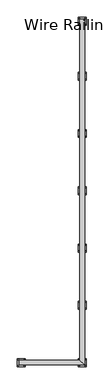
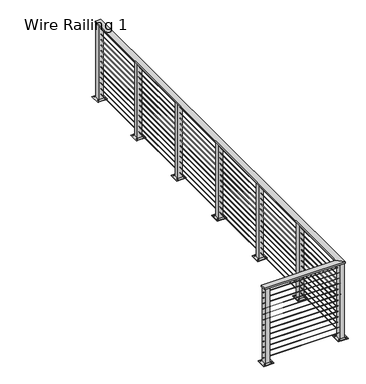
"""IFC4 building model written with IfcOpenShell, lengths in millimetres: railing geometry, Wire Railing 1."""

from ifc_helpers import new_model, si_unit, point, frame, frame_2d, origin, place, context, project, spatial, polyline, circle_curve, ellipse_curve, trimmed, segment, composite_curve, outline, extrude, faceted_brep, source, transform, mapped, element, save
from ifc_brep_helpers import plane_surface, cylinder_surface, advanced_brep


def wire_railing_1_7bc1b7ee(model_context):
    return source(origin(), model_context, "Body", "SolidModel", [
        faceted_brep([(33160.7531764, 36329.6332942, 267462.0), (33236.9531764, 36329.6332942, 267462.0), (33236.9531764, 36329.6332942, 267442.95), (33160.7531764, 36329.6332942, 267442.95), (33160.7531764, 30812.4406612, 267462.0), (33236.9531764, 30736.2406612, 267462.0), (33236.9531764, 30736.2406612, 267442.95), (33160.7531764, 30812.4406612, 267442.95), (32175.4465778, 30812.4406612, 267462.0), (32175.4465778, 30812.4406612, 267442.95), (32175.4465778, 30736.2406612, 267442.95), (32175.4465778, 30736.2406612, 267462.0)], [[[0, 1, 2, 3]], [[1, 0, 4, 5]], [[2, 1, 5, 6]], [[3, 2, 6, 7]], [[0, 3, 7, 4]], [[8, 9, 10, 11]], [[5, 4, 8, 11]], [[6, 5, 11, 10]], [[7, 6, 10, 9]], [[4, 7, 9, 8]]]),
        advanced_brep(
        [(33201.2344264, 36329.6332942, 267383.41875), (33196.4719264, 36329.6332942, 267383.41875), (33201.2344264, 30771.9594112, 267383.41875), (33196.4719264, 30776.7219112, 267383.41875), (32175.4465778, 30771.9594112, 267383.41875), (32175.4465778, 30776.7219112, 267383.41875)],
        [
            (0, 1, circle_curve(frame((33198.8531764, 36329.6332942, 267383.41875), z_axis=(0.0, 1.0, 0.0), x_axis=(-1.0, 0.0, 0.0)), 2.38125)),
            (1, 0, circle_curve(frame((33198.8531764, 36329.6332942, 267383.41875), z_axis=(0.0, 1.0, 0.0), x_axis=(-1.0, 0.0, 0.0)), 2.38125)),
            (0, 2),
            (2, 3, ellipse_curve(frame((33198.8531764, 30774.3406612, 267383.41875), z_axis=(0.7071067811865475, 0.7071067811865475, 0.0), x_axis=(-0.7071067811865474, 0.7071067811865476, 0.0)), 3.367596, 2.38125)),
            (3, 1),
            (3, 2, ellipse_curve(frame((33198.8531764, 30774.3406612, 267383.41875), z_axis=(0.7071067811865475, 0.7071067811865475, 0.0), x_axis=(-0.7071067811865474, 0.7071067811865476, 0.0)), 3.367596, 2.38125)),
            (4, 5, circle_curve(frame((32175.4465778, 30774.3406612, 267383.41875), z_axis=(-1.0, 0.0, 0.0), x_axis=(0.0, 1.0, 0.0)), 2.38125)),
            (5, 4, circle_curve(frame((32175.4465778, 30774.3406612, 267383.41875), z_axis=(-1.0, 0.0, 0.0), x_axis=(0.0, 1.0, 0.0)), 2.38125)),
            (2, 4),
            (5, 3),
        ],
        [
            plane_surface(frame((33198.8531764, 36329.6332942, 267385.8), z_axis=(0.0, 1.0, 0.0), x_axis=(0.0, 0.0, -1.0))),
            cylinder_surface(frame((33198.8531764, 36329.6332942, 267383.41875), z_axis=(0.0, 1.0, 0.0), x_axis=(-1.0, 0.0, 0.0)), 2.38125),
            plane_surface(frame((32175.4465778, 30774.3406612, 267385.8), z_axis=(-1.0, 0.0, 0.0), x_axis=(0.0, -1.0, 0.0))),
            cylinder_surface(frame((33198.8531764, 30774.3406612, 267383.41875), z_axis=(1.0, 0.0, 0.0), x_axis=(0.0, 1.0, 0.0)), 2.38125),
        ],
        [
            (0, [[1, 2]]),
            (1, [[-1, 3, 4, 5]]),
            (1, [[-2, -5, 6, -3]]),
            (2, [[7, 8]]),
            (3, [[-4, 9, -8, 10]]),
            (3, [[-6, -10, -7, -9]]),
        ],
    ),
        advanced_brep(
        [(33201.2344264, 36329.6332942, 267307.21875), (33196.4719264, 36329.6332942, 267307.21875), (33201.2344264, 30771.9594112, 267307.21875), (33196.4719264, 30776.7219112, 267307.21875), (32175.4465778, 30771.9594112, 267307.21875), (32175.4465778, 30776.7219112, 267307.21875)],
        [
            (0, 1, circle_curve(frame((33198.8531764, 36329.6332942, 267307.21875), z_axis=(0.0, 1.0, 0.0), x_axis=(-1.0, 0.0, 0.0)), 2.38125)),
            (1, 0, circle_curve(frame((33198.8531764, 36329.6332942, 267307.21875), z_axis=(0.0, 1.0, 0.0), x_axis=(-1.0, 0.0, 0.0)), 2.38125)),
            (0, 2),
            (2, 3, ellipse_curve(frame((33198.8531764, 30774.3406612, 267307.21875), z_axis=(0.7071067811865475, 0.7071067811865475, 0.0), x_axis=(-0.7071067811865474, 0.7071067811865476, 0.0)), 3.367596, 2.38125)),
            (3, 1),
            (3, 2, ellipse_curve(frame((33198.8531764, 30774.3406612, 267307.21875), z_axis=(0.7071067811865475, 0.7071067811865475, 0.0), x_axis=(-0.7071067811865474, 0.7071067811865476, 0.0)), 3.367596, 2.38125)),
            (4, 5, circle_curve(frame((32175.4465778, 30774.3406612, 267307.21875), z_axis=(-1.0, 0.0, 0.0), x_axis=(0.0, 1.0, 0.0)), 2.38125)),
            (5, 4, circle_curve(frame((32175.4465778, 30774.3406612, 267307.21875), z_axis=(-1.0, 0.0, 0.0), x_axis=(0.0, 1.0, 0.0)), 2.38125)),
            (2, 4),
            (5, 3),
        ],
        [
            plane_surface(frame((33198.8531764, 36329.6332942, 267309.6), z_axis=(0.0, 1.0, 0.0), x_axis=(0.0, 0.0, -1.0))),
            cylinder_surface(frame((33198.8531764, 36329.6332942, 267307.21875), z_axis=(0.0, 1.0, 0.0), x_axis=(-1.0, 0.0, 0.0)), 2.38125),
            plane_surface(frame((32175.4465778, 30774.3406612, 267309.6), z_axis=(-1.0, 0.0, 0.0), x_axis=(0.0, -1.0, 0.0))),
            cylinder_surface(frame((33198.8531764, 30774.3406612, 267307.21875), z_axis=(1.0, 0.0, 0.0), x_axis=(0.0, 1.0, 0.0)), 2.38125),
        ],
        [
            (0, [[1, 2]]),
            (1, [[-1, 3, 4, 5]]),
            (1, [[-2, -5, 6, -3]]),
            (2, [[7, 8]]),
            (3, [[-4, 9, -8, 10]]),
            (3, [[-6, -10, -7, -9]]),
        ],
    ),
        advanced_brep(
        [(33201.2344264, 36329.6332942, 267231.01875), (33196.4719264, 36329.6332942, 267231.01875), (33201.2344264, 30771.9594112, 267231.01875), (33196.4719264, 30776.7219112, 267231.01875), (32175.4465778, 30771.9594112, 267231.01875), (32175.4465778, 30776.7219112, 267231.01875)],
        [
            (0, 1, circle_curve(frame((33198.8531764, 36329.6332942, 267231.01875), z_axis=(0.0, 1.0, 0.0), x_axis=(-1.0, 0.0, 0.0)), 2.38125)),
            (1, 0, circle_curve(frame((33198.8531764, 36329.6332942, 267231.01875), z_axis=(0.0, 1.0, 0.0), x_axis=(-1.0, 0.0, 0.0)), 2.38125)),
            (0, 2),
            (2, 3, ellipse_curve(frame((33198.8531764, 30774.3406612, 267231.01875), z_axis=(0.7071067811865475, 0.7071067811865475, 0.0), x_axis=(-0.7071067811865474, 0.7071067811865476, 0.0)), 3.367596, 2.38125)),
            (3, 1),
            (3, 2, ellipse_curve(frame((33198.8531764, 30774.3406612, 267231.01875), z_axis=(0.7071067811865475, 0.7071067811865475, 0.0), x_axis=(-0.7071067811865474, 0.7071067811865476, 0.0)), 3.367596, 2.38125)),
            (4, 5, circle_curve(frame((32175.4465778, 30774.3406612, 267231.01875), z_axis=(-1.0, 0.0, 0.0), x_axis=(0.0, 1.0, 0.0)), 2.38125)),
            (5, 4, circle_curve(frame((32175.4465778, 30774.3406612, 267231.01875), z_axis=(-1.0, 0.0, 0.0), x_axis=(0.0, 1.0, 0.0)), 2.38125)),
            (2, 4),
            (5, 3),
        ],
        [
            plane_surface(frame((33198.8531764, 36329.6332942, 267233.4), z_axis=(0.0, 1.0, 0.0), x_axis=(0.0, 0.0, -1.0))),
            cylinder_surface(frame((33198.8531764, 36329.6332942, 267231.01875), z_axis=(0.0, 1.0, 0.0), x_axis=(-1.0, 0.0, 0.0)), 2.38125),
            plane_surface(frame((32175.4465778, 30774.3406612, 267233.4), z_axis=(-1.0, 0.0, 0.0), x_axis=(0.0, -1.0, 0.0))),
            cylinder_surface(frame((33198.8531764, 30774.3406612, 267231.01875), z_axis=(1.0, 0.0, 0.0), x_axis=(0.0, 1.0, 0.0)), 2.38125),
        ],
        [
            (0, [[1, 2]]),
            (1, [[-1, 3, 4, 5]]),
            (1, [[-2, -5, 6, -3]]),
            (2, [[7, 8]]),
            (3, [[-4, 9, -8, 10]]),
            (3, [[-6, -10, -7, -9]]),
        ],
    ),
        advanced_brep(
        [(33201.2344264, 36329.6332942, 267154.81875), (33196.4719264, 36329.6332942, 267154.81875), (33201.2344264, 30771.9594112, 267154.81875), (33196.4719264, 30776.7219112, 267154.81875), (32175.4465778, 30771.9594112, 267154.81875), (32175.4465778, 30776.7219112, 267154.81875)],
        [
            (0, 1, circle_curve(frame((33198.8531764, 36329.6332942, 267154.81875), z_axis=(0.0, 1.0, 0.0), x_axis=(-1.0, 0.0, 0.0)), 2.38125)),
            (1, 0, circle_curve(frame((33198.8531764, 36329.6332942, 267154.81875), z_axis=(0.0, 1.0, 0.0), x_axis=(-1.0, 0.0, 0.0)), 2.38125)),
            (0, 2),
            (2, 3, ellipse_curve(frame((33198.8531764, 30774.3406612, 267154.81875), z_axis=(0.7071067811865475, 0.7071067811865475, 0.0), x_axis=(-0.7071067811865474, 0.7071067811865476, 0.0)), 3.367596, 2.38125)),
            (3, 1),
            (3, 2, ellipse_curve(frame((33198.8531764, 30774.3406612, 267154.81875), z_axis=(0.7071067811865475, 0.7071067811865475, 0.0), x_axis=(-0.7071067811865474, 0.7071067811865476, 0.0)), 3.367596, 2.38125)),
            (4, 5, circle_curve(frame((32175.4465778, 30774.3406612, 267154.81875), z_axis=(-1.0, 0.0, 0.0), x_axis=(0.0, 1.0, 0.0)), 2.38125)),
            (5, 4, circle_curve(frame((32175.4465778, 30774.3406612, 267154.81875), z_axis=(-1.0, 0.0, 0.0), x_axis=(0.0, 1.0, 0.0)), 2.38125)),
            (2, 4),
            (5, 3),
        ],
        [
            plane_surface(frame((33198.8531764, 36329.6332942, 267157.2), z_axis=(0.0, 1.0, 0.0), x_axis=(0.0, 0.0, -1.0))),
            cylinder_surface(frame((33198.8531764, 36329.6332942, 267154.81875), z_axis=(0.0, 1.0, 0.0), x_axis=(-1.0, 0.0, 0.0)), 2.38125),
            plane_surface(frame((32175.4465778, 30774.3406612, 267157.2), z_axis=(-1.0, 0.0, 0.0), x_axis=(0.0, -1.0, 0.0))),
            cylinder_surface(frame((33198.8531764, 30774.3406612, 267154.81875), z_axis=(1.0, 0.0, 0.0), x_axis=(0.0, 1.0, 0.0)), 2.38125),
        ],
        [
            (0, [[1, 2]]),
            (1, [[-1, 3, 4, 5]]),
            (1, [[-2, -5, 6, -3]]),
            (2, [[7, 8]]),
            (3, [[-4, 9, -8, 10]]),
            (3, [[-6, -10, -7, -9]]),
        ],
    ),
        advanced_brep(
        [(33201.2344264, 36329.6332942, 267078.61875), (33196.4719264, 36329.6332942, 267078.61875), (33201.2344264, 30771.9594112, 267078.61875), (33196.4719264, 30776.7219112, 267078.61875), (32175.4465778, 30771.9594112, 267078.61875), (32175.4465778, 30776.7219112, 267078.61875)],
        [
            (0, 1, circle_curve(frame((33198.8531764, 36329.6332942, 267078.61875), z_axis=(0.0, 1.0, 0.0), x_axis=(-1.0, 0.0, 0.0)), 2.38125)),
            (1, 0, circle_curve(frame((33198.8531764, 36329.6332942, 267078.61875), z_axis=(0.0, 1.0, 0.0), x_axis=(-1.0, 0.0, 0.0)), 2.38125)),
            (0, 2),
            (2, 3, ellipse_curve(frame((33198.8531764, 30774.3406612, 267078.61875), z_axis=(0.7071067811865475, 0.7071067811865475, 0.0), x_axis=(-0.7071067811865474, 0.7071067811865476, 0.0)), 3.367596, 2.38125)),
            (3, 1),
            (3, 2, ellipse_curve(frame((33198.8531764, 30774.3406612, 267078.61875), z_axis=(0.7071067811865475, 0.7071067811865475, 0.0), x_axis=(-0.7071067811865474, 0.7071067811865476, 0.0)), 3.367596, 2.38125)),
            (4, 5, circle_curve(frame((32175.4465778, 30774.3406612, 267078.61875), z_axis=(-1.0, 0.0, 0.0), x_axis=(0.0, 1.0, 0.0)), 2.38125)),
            (5, 4, circle_curve(frame((32175.4465778, 30774.3406612, 267078.61875), z_axis=(-1.0, 0.0, 0.0), x_axis=(0.0, 1.0, 0.0)), 2.38125)),
            (2, 4),
            (5, 3),
        ],
        [
            plane_surface(frame((33198.8531764, 36329.6332942, 267081.0), z_axis=(0.0, 1.0, 0.0), x_axis=(0.0, 0.0, -1.0))),
            cylinder_surface(frame((33198.8531764, 36329.6332942, 267078.61875), z_axis=(0.0, 1.0, 0.0), x_axis=(-1.0, 0.0, 0.0)), 2.38125),
            plane_surface(frame((32175.4465778, 30774.3406612, 267081.0), z_axis=(-1.0, 0.0, 0.0), x_axis=(0.0, -1.0, 0.0))),
            cylinder_surface(frame((33198.8531764, 30774.3406612, 267078.61875), z_axis=(1.0, 0.0, 0.0), x_axis=(0.0, 1.0, 0.0)), 2.38125),
        ],
        [
            (0, [[1, 2]]),
            (1, [[-1, 3, 4, 5]]),
            (1, [[-2, -5, 6, -3]]),
            (2, [[7, 8]]),
            (3, [[-4, 9, -8, 10]]),
            (3, [[-6, -10, -7, -9]]),
        ],
    ),
        advanced_brep(
        [(33201.2344264, 36329.6332942, 267002.41875), (33196.4719264, 36329.6332942, 267002.41875), (33201.2344264, 30771.9594112, 267002.41875), (33196.4719264, 30776.7219112, 267002.41875), (32175.4465778, 30771.9594112, 267002.41875), (32175.4465778, 30776.7219112, 267002.41875)],
        [
            (0, 1, circle_curve(frame((33198.8531764, 36329.6332942, 267002.41875), z_axis=(0.0, 1.0, 0.0), x_axis=(-1.0, 0.0, 0.0)), 2.38125)),
            (1, 0, circle_curve(frame((33198.8531764, 36329.6332942, 267002.41875), z_axis=(0.0, 1.0, 0.0), x_axis=(-1.0, 0.0, 0.0)), 2.38125)),
            (0, 2),
            (2, 3, ellipse_curve(frame((33198.8531764, 30774.3406612, 267002.41875), z_axis=(0.7071067811865475, 0.7071067811865475, 0.0), x_axis=(-0.7071067811865474, 0.7071067811865476, 0.0)), 3.367596, 2.38125)),
            (3, 1),
            (3, 2, ellipse_curve(frame((33198.8531764, 30774.3406612, 267002.41875), z_axis=(0.7071067811865475, 0.7071067811865475, 0.0), x_axis=(-0.7071067811865474, 0.7071067811865476, 0.0)), 3.367596, 2.38125)),
            (4, 5, circle_curve(frame((32175.4465778, 30774.3406612, 267002.41875), z_axis=(-1.0, 0.0, 0.0), x_axis=(0.0, 1.0, 0.0)), 2.38125)),
            (5, 4, circle_curve(frame((32175.4465778, 30774.3406612, 267002.41875), z_axis=(-1.0, 0.0, 0.0), x_axis=(0.0, 1.0, 0.0)), 2.38125)),
            (2, 4),
            (5, 3),
        ],
        [
            plane_surface(frame((33198.8531764, 36329.6332942, 267004.8), z_axis=(0.0, 1.0, 0.0), x_axis=(0.0, 0.0, -1.0))),
            cylinder_surface(frame((33198.8531764, 36329.6332942, 267002.41875), z_axis=(0.0, 1.0, 0.0), x_axis=(-1.0, 0.0, 0.0)), 2.38125),
            plane_surface(frame((32175.4465778, 30774.3406612, 267004.8), z_axis=(-1.0, 0.0, 0.0), x_axis=(0.0, -1.0, 0.0))),
            cylinder_surface(frame((33198.8531764, 30774.3406612, 267002.41875), z_axis=(1.0, 0.0, 0.0), x_axis=(0.0, 1.0, 0.0)), 2.38125),
        ],
        [
            (0, [[1, 2]]),
            (1, [[-1, 3, 4, 5]]),
            (1, [[-2, -5, 6, -3]]),
            (2, [[7, 8]]),
            (3, [[-4, 9, -8, 10]]),
            (3, [[-6, -10, -7, -9]]),
        ],
    ),
        advanced_brep(
        [(33201.2344264, 36329.6332942, 266926.21875), (33196.4719264, 36329.6332942, 266926.21875), (33201.2344264, 30771.9594112, 266926.21875), (33196.4719264, 30776.7219112, 266926.21875), (32175.4465778, 30771.9594112, 266926.21875), (32175.4465778, 30776.7219112, 266926.21875)],
        [
            (0, 1, circle_curve(frame((33198.8531764, 36329.6332942, 266926.21875), z_axis=(0.0, 1.0, 0.0), x_axis=(-1.0, 0.0, 0.0)), 2.38125)),
            (1, 0, circle_curve(frame((33198.8531764, 36329.6332942, 266926.21875), z_axis=(0.0, 1.0, 0.0), x_axis=(-1.0, 0.0, 0.0)), 2.38125)),
            (0, 2),
            (2, 3, ellipse_curve(frame((33198.8531764, 30774.3406612, 266926.21875), z_axis=(0.7071067811865475, 0.7071067811865475, 0.0), x_axis=(-0.7071067811865474, 0.7071067811865476, 0.0)), 3.367596, 2.38125)),
            (3, 1),
            (3, 2, ellipse_curve(frame((33198.8531764, 30774.3406612, 266926.21875), z_axis=(0.7071067811865475, 0.7071067811865475, 0.0), x_axis=(-0.7071067811865474, 0.7071067811865476, 0.0)), 3.367596, 2.38125)),
            (4, 5, circle_curve(frame((32175.4465778, 30774.3406612, 266926.21875), z_axis=(-1.0, 0.0, 0.0), x_axis=(0.0, 1.0, 0.0)), 2.38125)),
            (5, 4, circle_curve(frame((32175.4465778, 30774.3406612, 266926.21875), z_axis=(-1.0, 0.0, 0.0), x_axis=(0.0, 1.0, 0.0)), 2.38125)),
            (2, 4),
            (5, 3),
        ],
        [
            plane_surface(frame((33198.8531764, 36329.6332942, 266928.6), z_axis=(0.0, 1.0, 0.0), x_axis=(0.0, 0.0, -1.0))),
            cylinder_surface(frame((33198.8531764, 36329.6332942, 266926.21875), z_axis=(0.0, 1.0, 0.0), x_axis=(-1.0, 0.0, 0.0)), 2.38125),
            plane_surface(frame((32175.4465778, 30774.3406612, 266928.6), z_axis=(-1.0, 0.0, 0.0), x_axis=(0.0, -1.0, 0.0))),
            cylinder_surface(frame((33198.8531764, 30774.3406612, 266926.21875), z_axis=(1.0, 0.0, 0.0), x_axis=(0.0, 1.0, 0.0)), 2.38125),
        ],
        [
            (0, [[1, 2]]),
            (1, [[-1, 3, 4, 5]]),
            (1, [[-2, -5, 6, -3]]),
            (2, [[7, 8]]),
            (3, [[-4, 9, -8, 10]]),
            (3, [[-6, -10, -7, -9]]),
        ],
    ),
        advanced_brep(
        [(33201.2344264, 36329.6332942, 266850.01875), (33196.4719264, 36329.6332942, 266850.01875), (33201.2344264, 30771.9594112, 266850.01875), (33196.4719264, 30776.7219112, 266850.01875), (32175.4465778, 30771.9594112, 266850.01875), (32175.4465778, 30776.7219112, 266850.01875)],
        [
            (0, 1, circle_curve(frame((33198.8531764, 36329.6332942, 266850.01875), z_axis=(0.0, 1.0, 0.0), x_axis=(-1.0, 0.0, 0.0)), 2.38125)),
            (1, 0, circle_curve(frame((33198.8531764, 36329.6332942, 266850.01875), z_axis=(0.0, 1.0, 0.0), x_axis=(-1.0, 0.0, 0.0)), 2.38125)),
            (0, 2),
            (2, 3, ellipse_curve(frame((33198.8531764, 30774.3406612, 266850.01875), z_axis=(0.7071067811865475, 0.7071067811865475, 0.0), x_axis=(-0.7071067811865474, 0.7071067811865476, 0.0)), 3.367596, 2.38125)),
            (3, 1),
            (3, 2, ellipse_curve(frame((33198.8531764, 30774.3406612, 266850.01875), z_axis=(0.7071067811865475, 0.7071067811865475, 0.0), x_axis=(-0.7071067811865474, 0.7071067811865476, 0.0)), 3.367596, 2.38125)),
            (4, 5, circle_curve(frame((32175.4465778, 30774.3406612, 266850.01875), z_axis=(-1.0, 0.0, 0.0), x_axis=(0.0, 1.0, 0.0)), 2.38125)),
            (5, 4, circle_curve(frame((32175.4465778, 30774.3406612, 266850.01875), z_axis=(-1.0, 0.0, 0.0), x_axis=(0.0, 1.0, 0.0)), 2.38125)),
            (2, 4),
            (5, 3),
        ],
        [
            plane_surface(frame((33198.8531764, 36329.6332942, 266852.4), z_axis=(0.0, 1.0, 0.0), x_axis=(0.0, 0.0, -1.0))),
            cylinder_surface(frame((33198.8531764, 36329.6332942, 266850.01875), z_axis=(0.0, 1.0, 0.0), x_axis=(-1.0, 0.0, 0.0)), 2.38125),
            plane_surface(frame((32175.4465778, 30774.3406612, 266852.4), z_axis=(-1.0, 0.0, 0.0), x_axis=(0.0, -1.0, 0.0))),
            cylinder_surface(frame((33198.8531764, 30774.3406612, 266850.01875), z_axis=(1.0, 0.0, 0.0), x_axis=(0.0, 1.0, 0.0)), 2.38125),
        ],
        [
            (0, [[1, 2]]),
            (1, [[-1, 3, 4, 5]]),
            (1, [[-2, -5, 6, -3]]),
            (2, [[7, 8]]),
            (3, [[-4, 9, -8, 10]]),
            (3, [[-6, -10, -7, -9]]),
        ],
    ),
        advanced_brep(
        [(33201.2344264, 36329.6332942, 266773.81875), (33196.4719264, 36329.6332942, 266773.81875), (33201.2344264, 30771.9594112, 266773.81875), (33196.4719264, 30776.7219112, 266773.81875), (32175.4465778, 30771.9594112, 266773.81875), (32175.4465778, 30776.7219112, 266773.81875)],
        [
            (0, 1, circle_curve(frame((33198.8531764, 36329.6332942, 266773.81875), z_axis=(0.0, 1.0, 0.0), x_axis=(-1.0, 0.0, 0.0)), 2.38125)),
            (1, 0, circle_curve(frame((33198.8531764, 36329.6332942, 266773.81875), z_axis=(0.0, 1.0, 0.0), x_axis=(-1.0, 0.0, 0.0)), 2.38125)),
            (0, 2),
            (2, 3, ellipse_curve(frame((33198.8531764, 30774.3406612, 266773.81875), z_axis=(0.7071067811865475, 0.7071067811865475, 0.0), x_axis=(-0.7071067811865474, 0.7071067811865476, 0.0)), 3.367596, 2.38125)),
            (3, 1),
            (3, 2, ellipse_curve(frame((33198.8531764, 30774.3406612, 266773.81875), z_axis=(0.7071067811865475, 0.7071067811865475, 0.0), x_axis=(-0.7071067811865474, 0.7071067811865476, 0.0)), 3.367596, 2.38125)),
            (4, 5, circle_curve(frame((32175.4465778, 30774.3406612, 266773.81875), z_axis=(-1.0, 0.0, 0.0), x_axis=(0.0, 1.0, 0.0)), 2.38125)),
            (5, 4, circle_curve(frame((32175.4465778, 30774.3406612, 266773.81875), z_axis=(-1.0, 0.0, 0.0), x_axis=(0.0, 1.0, 0.0)), 2.38125)),
            (2, 4),
            (5, 3),
        ],
        [
            plane_surface(frame((33198.8531764, 36329.6332942, 266776.2), z_axis=(0.0, 1.0, 0.0), x_axis=(0.0, 0.0, -1.0))),
            cylinder_surface(frame((33198.8531764, 36329.6332942, 266773.81875), z_axis=(0.0, 1.0, 0.0), x_axis=(-1.0, 0.0, 0.0)), 2.38125),
            plane_surface(frame((32175.4465778, 30774.3406612, 266776.2), z_axis=(-1.0, 0.0, 0.0), x_axis=(0.0, -1.0, 0.0))),
            cylinder_surface(frame((33198.8531764, 30774.3406612, 266773.81875), z_axis=(1.0, 0.0, 0.0), x_axis=(0.0, 1.0, 0.0)), 2.38125),
        ],
        [
            (0, [[1, 2]]),
            (1, [[-1, 3, 4, 5]]),
            (1, [[-2, -5, 6, -3]]),
            (2, [[7, 8]]),
            (3, [[-4, 9, -8, 10]]),
            (3, [[-6, -10, -7, -9]]),
        ],
    ),
        advanced_brep(
        [(33201.2344264, 36329.6332942, 266697.61875), (33196.4719264, 36329.6332942, 266697.61875), (33201.2344264, 30771.9594112, 266697.61875), (33196.4719264, 30776.7219112, 266697.61875), (32175.4465778, 30771.9594112, 266697.61875), (32175.4465778, 30776.7219112, 266697.61875)],
        [
            (0, 1, circle_curve(frame((33198.8531764, 36329.6332942, 266697.61875), z_axis=(0.0, 1.0, 0.0), x_axis=(-1.0, 0.0, 0.0)), 2.38125)),
            (1, 0, circle_curve(frame((33198.8531764, 36329.6332942, 266697.61875), z_axis=(0.0, 1.0, 0.0), x_axis=(-1.0, 0.0, 0.0)), 2.38125)),
            (0, 2),
            (2, 3, ellipse_curve(frame((33198.8531764, 30774.3406612, 266697.61875), z_axis=(0.7071067811865475, 0.7071067811865475, 0.0), x_axis=(-0.7071067811865474, 0.7071067811865476, 0.0)), 3.367596, 2.38125)),
            (3, 1),
            (3, 2, ellipse_curve(frame((33198.8531764, 30774.3406612, 266697.61875), z_axis=(0.7071067811865475, 0.7071067811865475, 0.0), x_axis=(-0.7071067811865474, 0.7071067811865476, 0.0)), 3.367596, 2.38125)),
            (4, 5, circle_curve(frame((32175.4465778, 30774.3406612, 266697.61875), z_axis=(-1.0, 0.0, 0.0), x_axis=(0.0, 1.0, 0.0)), 2.38125)),
            (5, 4, circle_curve(frame((32175.4465778, 30774.3406612, 266697.61875), z_axis=(-1.0, 0.0, 0.0), x_axis=(0.0, 1.0, 0.0)), 2.38125)),
            (2, 4),
            (5, 3),
        ],
        [
            plane_surface(frame((33198.8531764, 36329.6332942, 266700.0), z_axis=(0.0, 1.0, 0.0), x_axis=(0.0, 0.0, -1.0))),
            cylinder_surface(frame((33198.8531764, 36329.6332942, 266697.61875), z_axis=(0.0, 1.0, 0.0), x_axis=(-1.0, 0.0, 0.0)), 2.38125),
            plane_surface(frame((32175.4465778, 30774.3406612, 266700.0), z_axis=(-1.0, 0.0, 0.0), x_axis=(0.0, -1.0, 0.0))),
            cylinder_surface(frame((33198.8531764, 30774.3406612, 266697.61875), z_axis=(1.0, 0.0, 0.0), x_axis=(0.0, 1.0, 0.0)), 2.38125),
        ],
        [
            (0, [[1, 2]]),
            (1, [[-1, 3, 4, 5]]),
            (1, [[-2, -5, 6, -3]]),
            (2, [[7, 8]]),
            (3, [[-4, 9, -8, 10]]),
            (3, [[-6, -10, -7, -9]]),
        ],
    ),
        advanced_brep(
        [(33201.2344264, 36329.6332942, 266621.41875), (33196.4719264, 36329.6332942, 266621.41875), (33201.2344264, 30771.9594112, 266621.41875), (33196.4719264, 30776.7219112, 266621.41875), (32175.4465778, 30771.9594112, 266621.41875), (32175.4465778, 30776.7219112, 266621.41875)],
        [
            (0, 1, circle_curve(frame((33198.8531764, 36329.6332942, 266621.41875), z_axis=(0.0, 1.0, 0.0), x_axis=(-1.0, 0.0, 0.0)), 2.38125)),
            (1, 0, circle_curve(frame((33198.8531764, 36329.6332942, 266621.41875), z_axis=(0.0, 1.0, 0.0), x_axis=(-1.0, 0.0, 0.0)), 2.38125)),
            (0, 2),
            (2, 3, ellipse_curve(frame((33198.8531764, 30774.3406612, 266621.41875), z_axis=(0.7071067811865475, 0.7071067811865475, 0.0), x_axis=(-0.7071067811865474, 0.7071067811865476, 0.0)), 3.367596, 2.38125)),
            (3, 1),
            (3, 2, ellipse_curve(frame((33198.8531764, 30774.3406612, 266621.41875), z_axis=(0.7071067811865475, 0.7071067811865475, 0.0), x_axis=(-0.7071067811865474, 0.7071067811865476, 0.0)), 3.367596, 2.38125)),
            (4, 5, circle_curve(frame((32175.4465778, 30774.3406612, 266621.41875), z_axis=(-1.0, 0.0, 0.0), x_axis=(0.0, 1.0, 0.0)), 2.38125)),
            (5, 4, circle_curve(frame((32175.4465778, 30774.3406612, 266621.41875), z_axis=(-1.0, 0.0, 0.0), x_axis=(0.0, 1.0, 0.0)), 2.38125)),
            (2, 4),
            (5, 3),
        ],
        [
            plane_surface(frame((33198.8531764, 36329.6332942, 266623.8), z_axis=(0.0, 1.0, 0.0), x_axis=(0.0, 0.0, -1.0))),
            cylinder_surface(frame((33198.8531764, 36329.6332942, 266621.41875), z_axis=(0.0, 1.0, 0.0), x_axis=(-1.0, 0.0, 0.0)), 2.38125),
            plane_surface(frame((32175.4465778, 30774.3406612, 266623.8), z_axis=(-1.0, 0.0, 0.0), x_axis=(0.0, -1.0, 0.0))),
            cylinder_surface(frame((33198.8531764, 30774.3406612, 266621.41875), z_axis=(1.0, 0.0, 0.0), x_axis=(0.0, 1.0, 0.0)), 2.38125),
        ],
        [
            (0, [[1, 2]]),
            (1, [[-1, 3, 4, 5]]),
            (1, [[-2, -5, 6, -3]]),
            (2, [[7, 8]]),
            (3, [[-4, 9, -8, 10]]),
            (3, [[-6, -10, -7, -9]]),
        ],
    ),
        advanced_brep(
        [(33201.2344264, 36329.6332942, 266545.21875), (33196.4719264, 36329.6332942, 266545.21875), (33201.2344264, 30771.9594112, 266545.21875), (33196.4719264, 30776.7219112, 266545.21875), (32175.4465778, 30771.9594112, 266545.21875), (32175.4465778, 30776.7219112, 266545.21875)],
        [
            (0, 1, circle_curve(frame((33198.8531764, 36329.6332942, 266545.21875), z_axis=(0.0, 1.0, 0.0), x_axis=(-1.0, 0.0, 0.0)), 2.38125)),
            (1, 0, circle_curve(frame((33198.8531764, 36329.6332942, 266545.21875), z_axis=(0.0, 1.0, 0.0), x_axis=(-1.0, 0.0, 0.0)), 2.38125)),
            (0, 2),
            (2, 3, ellipse_curve(frame((33198.8531764, 30774.3406612, 266545.21875), z_axis=(0.7071067811865475, 0.7071067811865475, 0.0), x_axis=(-0.7071067811865474, 0.7071067811865476, 0.0)), 3.367596, 2.38125)),
            (3, 1),
            (3, 2, ellipse_curve(frame((33198.8531764, 30774.3406612, 266545.21875), z_axis=(0.7071067811865475, 0.7071067811865475, 0.0), x_axis=(-0.7071067811865474, 0.7071067811865476, 0.0)), 3.367596, 2.38125)),
            (4, 5, circle_curve(frame((32175.4465778, 30774.3406612, 266545.21875), z_axis=(-1.0, 0.0, 0.0), x_axis=(0.0, 1.0, 0.0)), 2.38125)),
            (5, 4, circle_curve(frame((32175.4465778, 30774.3406612, 266545.21875), z_axis=(-1.0, 0.0, 0.0), x_axis=(0.0, 1.0, 0.0)), 2.38125)),
            (2, 4),
            (5, 3),
        ],
        [
            plane_surface(frame((33198.8531764, 36329.6332942, 266547.6), z_axis=(0.0, 1.0, 0.0), x_axis=(0.0, 0.0, -1.0))),
            cylinder_surface(frame((33198.8531764, 36329.6332942, 266545.21875), z_axis=(0.0, 1.0, 0.0), x_axis=(-1.0, 0.0, 0.0)), 2.38125),
            plane_surface(frame((32175.4465778, 30774.3406612, 266547.6), z_axis=(-1.0, 0.0, 0.0), x_axis=(0.0, -1.0, 0.0))),
            cylinder_surface(frame((33198.8531764, 30774.3406612, 266545.21875), z_axis=(1.0, 0.0, 0.0), x_axis=(0.0, 1.0, 0.0)), 2.38125),
        ],
        [
            (0, [[1, 2]]),
            (1, [[-1, 3, 4, 5]]),
            (1, [[-2, -5, 6, -3]]),
            (2, [[7, 8]]),
            (3, [[-4, 9, -8, 10]]),
            (3, [[-6, -10, -7, -9]]),
        ],
    ),
        advanced_brep(
        [(33201.2344264, 36329.6332942, 266469.01875), (33196.4719264, 36329.6332942, 266469.01875), (33201.2344264, 30771.9594112, 266469.01875), (33196.4719264, 30776.7219112, 266469.01875), (32175.4465778, 30771.9594112, 266469.01875), (32175.4465778, 30776.7219112, 266469.01875)],
        [
            (0, 1, circle_curve(frame((33198.8531764, 36329.6332942, 266469.01875), z_axis=(0.0, 1.0, 0.0), x_axis=(-1.0, 0.0, 0.0)), 2.38125)),
            (1, 0, circle_curve(frame((33198.8531764, 36329.6332942, 266469.01875), z_axis=(0.0, 1.0, 0.0), x_axis=(-1.0, 0.0, 0.0)), 2.38125)),
            (0, 2),
            (2, 3, ellipse_curve(frame((33198.8531764, 30774.3406612, 266469.01875), z_axis=(0.7071067811865475, 0.7071067811865475, 0.0), x_axis=(-0.7071067811865474, 0.7071067811865476, 0.0)), 3.367596, 2.38125)),
            (3, 1),
            (3, 2, ellipse_curve(frame((33198.8531764, 30774.3406612, 266469.01875), z_axis=(0.7071067811865475, 0.7071067811865475, 0.0), x_axis=(-0.7071067811865474, 0.7071067811865476, 0.0)), 3.367596, 2.38125)),
            (4, 5, circle_curve(frame((32175.4465778, 30774.3406612, 266469.01875), z_axis=(-1.0, 0.0, 0.0), x_axis=(0.0, 1.0, 0.0)), 2.38125)),
            (5, 4, circle_curve(frame((32175.4465778, 30774.3406612, 266469.01875), z_axis=(-1.0, 0.0, 0.0), x_axis=(0.0, 1.0, 0.0)), 2.38125)),
            (2, 4),
            (5, 3),
        ],
        [
            plane_surface(frame((33198.8531764, 36329.6332942, 266471.4), z_axis=(0.0, 1.0, 0.0), x_axis=(0.0, 0.0, -1.0))),
            cylinder_surface(frame((33198.8531764, 36329.6332942, 266469.01875), z_axis=(0.0, 1.0, 0.0), x_axis=(-1.0, 0.0, 0.0)), 2.38125),
            plane_surface(frame((32175.4465778, 30774.3406612, 266471.4), z_axis=(-1.0, 0.0, 0.0), x_axis=(0.0, -1.0, 0.0))),
            cylinder_surface(frame((33198.8531764, 30774.3406612, 266469.01875), z_axis=(1.0, 0.0, 0.0), x_axis=(0.0, 1.0, 0.0)), 2.38125),
        ],
        [
            (0, [[1, 2]]),
            (1, [[-1, 3, 4, 5]]),
            (1, [[-2, -5, 6, -3]]),
            (2, [[7, 8]]),
            (3, [[-4, 9, -8, 10]]),
            (3, [[-6, -10, -7, -9]]),
        ],
    ),
        extrude(outline(composite_curve([segment(trimmed(circle_curve(frame_2d((33154.4031764, 31744.6727667)), 6.35), [point((33148.0531764, 31744.6727667))], [point((33160.7531764, 31744.6727667))], False, "CARTESIAN"), True, "CONTINUOUS"), segment(trimmed(circle_curve(frame_2d((33154.4031764, 31744.6727667)), 6.35), [point((33160.7531764, 31744.6727667))], [point((33148.0531764, 31744.6727667))], False, "CARTESIAN"), True, "CONTINUOUS")], self_intersect=False)), frame((0.0, 0.0, 266395.2), z_axis=(0.0, 0.0, 1.0), x_axis=(1.0, 0.0, 0.0)), (0.0, 0.0, 1.0), 12.7),
        extrude(outline(composite_curve([segment(trimmed(circle_curve(frame_2d((33243.3031764, 31744.6727667)), 6.35), [point((33236.9531764, 31744.6727667))], [point((33249.6531764, 31744.6727667))], False, "CARTESIAN"), True, "CONTINUOUS"), segment(trimmed(circle_curve(frame_2d((33243.3031764, 31744.6727667)), 6.35), [point((33249.6531764, 31744.6727667))], [point((33236.9531764, 31744.6727667))], False, "CARTESIAN"), True, "CONTINUOUS")], self_intersect=False)), frame((0.0, 0.0, 266395.2), z_axis=(0.0, 0.0, 1.0), x_axis=(1.0, 0.0, 0.0)), (0.0, 0.0, 1.0), 12.7),
        extrude(outline(composite_curve([segment(trimmed(circle_curve(frame_2d((33154.4031764, 31655.7727667)), 6.35), [point((33148.0531764, 31655.7727667))], [point((33160.7531764, 31655.7727667))], False, "CARTESIAN"), True, "CONTINUOUS"), segment(trimmed(circle_curve(frame_2d((33154.4031764, 31655.7727667)), 6.35), [point((33160.7531764, 31655.7727667))], [point((33148.0531764, 31655.7727667))], False, "CARTESIAN"), True, "CONTINUOUS")], self_intersect=False)), frame((0.0, 0.0, 266395.2), z_axis=(0.0, 0.0, 1.0), x_axis=(1.0, 0.0, 0.0)), (0.0, 0.0, 1.0), 12.7),
        extrude(outline(composite_curve([segment(trimmed(circle_curve(frame_2d((33243.3031764, 31655.7727667)), 6.35), [point((33236.9531764, 31655.7727667))], [point((33249.6531764, 31655.7727667))], False, "CARTESIAN"), True, "CONTINUOUS"), segment(trimmed(circle_curve(frame_2d((33243.3031764, 31655.7727667)), 6.35), [point((33249.6531764, 31655.7727667))], [point((33236.9531764, 31655.7727667))], False, "CARTESIAN"), True, "CONTINUOUS")], self_intersect=False)), frame((0.0, 0.0, 266395.2), z_axis=(0.0, 0.0, 1.0), x_axis=(1.0, 0.0, 0.0)), (0.0, 0.0, 1.0), 12.7),
        extrude(outline(polyline([(33262.3531764, 31763.7227667), (33262.3531764, 31636.7227667), (33135.3531764, 31636.7227667), (33135.3531764, 31763.7227667), (33262.3531764, 31763.7227667)])), frame((0.0, 0.0, 266395.2), z_axis=(0.0, 0.0, 1.0), x_axis=(1.0, 0.0, 0.0)), (0.0, 0.0, 1.0), 6.35),
        extrude(outline(polyline([(33229.0156764, 31730.3852667), (33229.0156764, 31670.0602667), (33168.6906764, 31670.0602667), (33168.6906764, 31730.3852667), (33229.0156764, 31730.3852667)]), holes=[polyline([(33222.6656764, 31724.0352667), (33175.0406764, 31724.0352667), (33175.0406764, 31676.4102667), (33222.6656764, 31676.4102667), (33222.6656764, 31724.0352667)])]), frame((0.0, 0.0, 266395.2), z_axis=(0.0, 0.0, 1.0), x_axis=(1.0, 0.0, 0.0)), (0.0, 0.0, 1.0), 1047.75),
        extrude(outline(composite_curve([segment(trimmed(circle_curve(frame_2d((33154.4031764, 32670.5548722)), 6.35), [point((33148.0531764, 32670.5548722))], [point((33160.7531764, 32670.5548722))], False, "CARTESIAN"), True, "CONTINUOUS"), segment(trimmed(circle_curve(frame_2d((33154.4031764, 32670.5548722)), 6.35), [point((33160.7531764, 32670.5548722))], [point((33148.0531764, 32670.5548722))], False, "CARTESIAN"), True, "CONTINUOUS")], self_intersect=False)), frame((0.0, 0.0, 266395.2), z_axis=(0.0, 0.0, 1.0), x_axis=(1.0, 0.0, 0.0)), (0.0, 0.0, 1.0), 12.7),
        extrude(outline(composite_curve([segment(trimmed(circle_curve(frame_2d((33243.3031764, 32670.5548722)), 6.35), [point((33236.9531764, 32670.5548722))], [point((33249.6531764, 32670.5548722))], False, "CARTESIAN"), True, "CONTINUOUS"), segment(trimmed(circle_curve(frame_2d((33243.3031764, 32670.5548722)), 6.35), [point((33249.6531764, 32670.5548722))], [point((33236.9531764, 32670.5548722))], False, "CARTESIAN"), True, "CONTINUOUS")], self_intersect=False)), frame((0.0, 0.0, 266395.2), z_axis=(0.0, 0.0, 1.0), x_axis=(1.0, 0.0, 0.0)), (0.0, 0.0, 1.0), 12.7),
        extrude(outline(composite_curve([segment(trimmed(circle_curve(frame_2d((33154.4031764, 32581.6548722)), 6.35), [point((33148.0531764, 32581.6548722))], [point((33160.7531764, 32581.6548722))], False, "CARTESIAN"), True, "CONTINUOUS"), segment(trimmed(circle_curve(frame_2d((33154.4031764, 32581.6548722)), 6.35), [point((33160.7531764, 32581.6548722))], [point((33148.0531764, 32581.6548722))], False, "CARTESIAN"), True, "CONTINUOUS")], self_intersect=False)), frame((0.0, 0.0, 266395.2), z_axis=(0.0, 0.0, 1.0), x_axis=(1.0, 0.0, 0.0)), (0.0, 0.0, 1.0), 12.7),
        extrude(outline(composite_curve([segment(trimmed(circle_curve(frame_2d((33243.3031764, 32581.6548722)), 6.35), [point((33236.9531764, 32581.6548722))], [point((33249.6531764, 32581.6548722))], False, "CARTESIAN"), True, "CONTINUOUS"), segment(trimmed(circle_curve(frame_2d((33243.3031764, 32581.6548722)), 6.35), [point((33249.6531764, 32581.6548722))], [point((33236.9531764, 32581.6548722))], False, "CARTESIAN"), True, "CONTINUOUS")], self_intersect=False)), frame((0.0, 0.0, 266395.2), z_axis=(0.0, 0.0, 1.0), x_axis=(1.0, 0.0, 0.0)), (0.0, 0.0, 1.0), 12.7),
        extrude(outline(polyline([(33262.3531764, 32689.6048722), (33262.3531764, 32562.6048722), (33135.3531764, 32562.6048722), (33135.3531764, 32689.6048722), (33262.3531764, 32689.6048722)])), frame((0.0, 0.0, 266395.2), z_axis=(0.0, 0.0, 1.0), x_axis=(1.0, 0.0, 0.0)), (0.0, 0.0, 1.0), 6.35),
        extrude(outline(polyline([(33229.0156764, 32656.2673722), (33229.0156764, 32595.9423722), (33168.6906764, 32595.9423722), (33168.6906764, 32656.2673722), (33229.0156764, 32656.2673722)]), holes=[polyline([(33222.6656764, 32649.9173722), (33175.0406764, 32649.9173722), (33175.0406764, 32602.2923722), (33222.6656764, 32602.2923722), (33222.6656764, 32649.9173722)])]), frame((0.0, 0.0, 266395.2), z_axis=(0.0, 0.0, 1.0), x_axis=(1.0, 0.0, 0.0)), (0.0, 0.0, 1.0), 1047.75),
        extrude(outline(composite_curve([segment(trimmed(circle_curve(frame_2d((33154.4031764, 33596.4369777)), 6.35), [point((33148.0531764, 33596.4369777))], [point((33160.7531764, 33596.4369777))], False, "CARTESIAN"), True, "CONTINUOUS"), segment(trimmed(circle_curve(frame_2d((33154.4031764, 33596.4369777)), 6.35), [point((33160.7531764, 33596.4369777))], [point((33148.0531764, 33596.4369777))], False, "CARTESIAN"), True, "CONTINUOUS")], self_intersect=False)), frame((0.0, 0.0, 266395.2), z_axis=(0.0, 0.0, 1.0), x_axis=(1.0, 0.0, 0.0)), (0.0, 0.0, 1.0), 12.7),
        extrude(outline(composite_curve([segment(trimmed(circle_curve(frame_2d((33243.3031764, 33596.4369777)), 6.35), [point((33236.9531764, 33596.4369777))], [point((33249.6531764, 33596.4369777))], False, "CARTESIAN"), True, "CONTINUOUS"), segment(trimmed(circle_curve(frame_2d((33243.3031764, 33596.4369777)), 6.35), [point((33249.6531764, 33596.4369777))], [point((33236.9531764, 33596.4369777))], False, "CARTESIAN"), True, "CONTINUOUS")], self_intersect=False)), frame((0.0, 0.0, 266395.2), z_axis=(0.0, 0.0, 1.0), x_axis=(1.0, 0.0, 0.0)), (0.0, 0.0, 1.0), 12.7),
        extrude(outline(composite_curve([segment(trimmed(circle_curve(frame_2d((33154.4031764, 33507.5369777)), 6.35), [point((33148.0531764, 33507.5369777))], [point((33160.7531764, 33507.5369777))], False, "CARTESIAN"), True, "CONTINUOUS"), segment(trimmed(circle_curve(frame_2d((33154.4031764, 33507.5369777)), 6.35), [point((33160.7531764, 33507.5369777))], [point((33148.0531764, 33507.5369777))], False, "CARTESIAN"), True, "CONTINUOUS")], self_intersect=False)), frame((0.0, 0.0, 266395.2), z_axis=(0.0, 0.0, 1.0), x_axis=(1.0, 0.0, 0.0)), (0.0, 0.0, 1.0), 12.7),
        extrude(outline(composite_curve([segment(trimmed(circle_curve(frame_2d((33243.3031764, 33507.5369777)), 6.35), [point((33236.9531764, 33507.5369777))], [point((33249.6531764, 33507.5369777))], False, "CARTESIAN"), True, "CONTINUOUS"), segment(trimmed(circle_curve(frame_2d((33243.3031764, 33507.5369777)), 6.35), [point((33249.6531764, 33507.5369777))], [point((33236.9531764, 33507.5369777))], False, "CARTESIAN"), True, "CONTINUOUS")], self_intersect=False)), frame((0.0, 0.0, 266395.2), z_axis=(0.0, 0.0, 1.0), x_axis=(1.0, 0.0, 0.0)), (0.0, 0.0, 1.0), 12.7),
        extrude(outline(polyline([(33262.3531764, 33615.4869777), (33262.3531764, 33488.4869777), (33135.3531764, 33488.4869777), (33135.3531764, 33615.4869777), (33262.3531764, 33615.4869777)])), frame((0.0, 0.0, 266395.2), z_axis=(0.0, 0.0, 1.0), x_axis=(1.0, 0.0, 0.0)), (0.0, 0.0, 1.0), 6.35),
        extrude(outline(polyline([(33229.0156764, 33582.1494777), (33229.0156764, 33521.8244777), (33168.6906764, 33521.8244777), (33168.6906764, 33582.1494777), (33229.0156764, 33582.1494777)]), holes=[polyline([(33222.6656764, 33575.7994777), (33175.0406764, 33575.7994777), (33175.0406764, 33528.1744777), (33222.6656764, 33528.1744777), (33222.6656764, 33575.7994777)])]), frame((0.0, 0.0, 266395.2), z_axis=(0.0, 0.0, 1.0), x_axis=(1.0, 0.0, 0.0)), (0.0, 0.0, 1.0), 1047.75),
        extrude(outline(composite_curve([segment(trimmed(circle_curve(frame_2d((33154.4031764, 34522.3190832)), 6.35), [point((33148.0531764, 34522.3190832))], [point((33160.7531764, 34522.3190832))], False, "CARTESIAN"), True, "CONTINUOUS"), segment(trimmed(circle_curve(frame_2d((33154.4031764, 34522.3190832)), 6.35), [point((33160.7531764, 34522.3190832))], [point((33148.0531764, 34522.3190832))], False, "CARTESIAN"), True, "CONTINUOUS")], self_intersect=False)), frame((0.0, 0.0, 266395.2), z_axis=(0.0, 0.0, 1.0), x_axis=(1.0, 0.0, 0.0)), (0.0, 0.0, 1.0), 12.7),
        extrude(outline(composite_curve([segment(trimmed(circle_curve(frame_2d((33243.3031764, 34522.3190832)), 6.35), [point((33236.9531764, 34522.3190832))], [point((33249.6531764, 34522.3190832))], False, "CARTESIAN"), True, "CONTINUOUS"), segment(trimmed(circle_curve(frame_2d((33243.3031764, 34522.3190832)), 6.35), [point((33249.6531764, 34522.3190832))], [point((33236.9531764, 34522.3190832))], False, "CARTESIAN"), True, "CONTINUOUS")], self_intersect=False)), frame((0.0, 0.0, 266395.2), z_axis=(0.0, 0.0, 1.0), x_axis=(1.0, 0.0, 0.0)), (0.0, 0.0, 1.0), 12.7),
        extrude(outline(composite_curve([segment(trimmed(circle_curve(frame_2d((33154.4031764, 34433.4190832)), 6.35), [point((33148.0531764, 34433.4190832))], [point((33160.7531764, 34433.4190832))], False, "CARTESIAN"), True, "CONTINUOUS"), segment(trimmed(circle_curve(frame_2d((33154.4031764, 34433.4190832)), 6.35), [point((33160.7531764, 34433.4190832))], [point((33148.0531764, 34433.4190832))], False, "CARTESIAN"), True, "CONTINUOUS")], self_intersect=False)), frame((0.0, 0.0, 266395.2), z_axis=(0.0, 0.0, 1.0), x_axis=(1.0, 0.0, 0.0)), (0.0, 0.0, 1.0), 12.7),
        extrude(outline(composite_curve([segment(trimmed(circle_curve(frame_2d((33243.3031764, 34433.4190832)), 6.35), [point((33236.9531764, 34433.4190832))], [point((33249.6531764, 34433.4190832))], False, "CARTESIAN"), True, "CONTINUOUS"), segment(trimmed(circle_curve(frame_2d((33243.3031764, 34433.4190832)), 6.35), [point((33249.6531764, 34433.4190832))], [point((33236.9531764, 34433.4190832))], False, "CARTESIAN"), True, "CONTINUOUS")], self_intersect=False)), frame((0.0, 0.0, 266395.2), z_axis=(0.0, 0.0, 1.0), x_axis=(1.0, 0.0, 0.0)), (0.0, 0.0, 1.0), 12.7),
        extrude(outline(polyline([(33262.3531764, 34541.3690832), (33262.3531764, 34414.3690832), (33135.3531764, 34414.3690832), (33135.3531764, 34541.3690832), (33262.3531764, 34541.3690832)])), frame((0.0, 0.0, 266395.2), z_axis=(0.0, 0.0, 1.0), x_axis=(1.0, 0.0, 0.0)), (0.0, 0.0, 1.0), 6.35),
        extrude(outline(polyline([(33229.0156764, 34508.0315832), (33229.0156764, 34447.7065832), (33168.6906764, 34447.7065832), (33168.6906764, 34508.0315832), (33229.0156764, 34508.0315832)]), holes=[polyline([(33222.6656764, 34501.6815832), (33175.0406764, 34501.6815832), (33175.0406764, 34454.0565832), (33222.6656764, 34454.0565832), (33222.6656764, 34501.6815832)])]), frame((0.0, 0.0, 266395.2), z_axis=(0.0, 0.0, 1.0), x_axis=(1.0, 0.0, 0.0)), (0.0, 0.0, 1.0), 1047.75),
        extrude(outline(composite_curve([segment(trimmed(circle_curve(frame_2d((33154.4031764, 35448.2011887)), 6.35), [point((33148.0531764, 35448.2011887))], [point((33160.7531764, 35448.2011887))], False, "CARTESIAN"), True, "CONTINUOUS"), segment(trimmed(circle_curve(frame_2d((33154.4031764, 35448.2011887)), 6.35), [point((33160.7531764, 35448.2011887))], [point((33148.0531764, 35448.2011887))], False, "CARTESIAN"), True, "CONTINUOUS")], self_intersect=False)), frame((0.0, 0.0, 266395.2), z_axis=(0.0, 0.0, 1.0), x_axis=(1.0, 0.0, 0.0)), (0.0, 0.0, 1.0), 12.7),
        extrude(outline(composite_curve([segment(trimmed(circle_curve(frame_2d((33243.3031764, 35448.2011887)), 6.35), [point((33236.9531764, 35448.2011887))], [point((33249.6531764, 35448.2011887))], False, "CARTESIAN"), True, "CONTINUOUS"), segment(trimmed(circle_curve(frame_2d((33243.3031764, 35448.2011887)), 6.35), [point((33249.6531764, 35448.2011887))], [point((33236.9531764, 35448.2011887))], False, "CARTESIAN"), True, "CONTINUOUS")], self_intersect=False)), frame((0.0, 0.0, 266395.2), z_axis=(0.0, 0.0, 1.0), x_axis=(1.0, 0.0, 0.0)), (0.0, 0.0, 1.0), 12.7),
        extrude(outline(composite_curve([segment(trimmed(circle_curve(frame_2d((33154.4031764, 35359.3011887)), 6.35), [point((33148.0531764, 35359.3011887))], [point((33160.7531764, 35359.3011887))], False, "CARTESIAN"), True, "CONTINUOUS"), segment(trimmed(circle_curve(frame_2d((33154.4031764, 35359.3011887)), 6.35), [point((33160.7531764, 35359.3011887))], [point((33148.0531764, 35359.3011887))], False, "CARTESIAN"), True, "CONTINUOUS")], self_intersect=False)), frame((0.0, 0.0, 266395.2), z_axis=(0.0, 0.0, 1.0), x_axis=(1.0, 0.0, 0.0)), (0.0, 0.0, 1.0), 12.7),
        extrude(outline(composite_curve([segment(trimmed(circle_curve(frame_2d((33243.3031764, 35359.3011887)), 6.35), [point((33236.9531764, 35359.3011887))], [point((33249.6531764, 35359.3011887))], False, "CARTESIAN"), True, "CONTINUOUS"), segment(trimmed(circle_curve(frame_2d((33243.3031764, 35359.3011887)), 6.35), [point((33249.6531764, 35359.3011887))], [point((33236.9531764, 35359.3011887))], False, "CARTESIAN"), True, "CONTINUOUS")], self_intersect=False)), frame((0.0, 0.0, 266395.2), z_axis=(0.0, 0.0, 1.0), x_axis=(1.0, 0.0, 0.0)), (0.0, 0.0, 1.0), 12.7),
        extrude(outline(polyline([(33262.3531764, 35467.2511887), (33262.3531764, 35340.2511887), (33135.3531764, 35340.2511887), (33135.3531764, 35467.2511887), (33262.3531764, 35467.2511887)])), frame((0.0, 0.0, 266395.2), z_axis=(0.0, 0.0, 1.0), x_axis=(1.0, 0.0, 0.0)), (0.0, 0.0, 1.0), 6.35),
        extrude(outline(polyline([(33229.0156764, 35433.9136887), (33229.0156764, 35373.5886887), (33168.6906764, 35373.5886887), (33168.6906764, 35433.9136887), (33229.0156764, 35433.9136887)]), holes=[polyline([(33222.6656764, 35427.5636887), (33175.0406764, 35427.5636887), (33175.0406764, 35379.9386887), (33222.6656764, 35379.9386887), (33222.6656764, 35427.5636887)])]), frame((0.0, 0.0, 266395.2), z_axis=(0.0, 0.0, 1.0), x_axis=(1.0, 0.0, 0.0)), (0.0, 0.0, 1.0), 1047.75),
        extrude(outline(composite_curve([segment(trimmed(circle_curve(frame_2d((33154.4031764, 30818.7906612)), 6.35), [point((33148.0531764, 30818.7906612))], [point((33160.7531764, 30818.7906612))], False, "CARTESIAN"), True, "CONTINUOUS"), segment(trimmed(circle_curve(frame_2d((33154.4031764, 30818.7906612)), 6.35), [point((33160.7531764, 30818.7906612))], [point((33148.0531764, 30818.7906612))], False, "CARTESIAN"), True, "CONTINUOUS")], self_intersect=False)), frame((0.0, 0.0, 266395.2), z_axis=(0.0, 0.0, 1.0), x_axis=(1.0, 0.0, 0.0)), (0.0, 0.0, 1.0), 12.7),
        extrude(outline(composite_curve([segment(trimmed(circle_curve(frame_2d((33243.3031764, 30818.7906612)), 6.35), [point((33236.9531764, 30818.7906612))], [point((33249.6531764, 30818.7906612))], False, "CARTESIAN"), True, "CONTINUOUS"), segment(trimmed(circle_curve(frame_2d((33243.3031764, 30818.7906612)), 6.35), [point((33249.6531764, 30818.7906612))], [point((33236.9531764, 30818.7906612))], False, "CARTESIAN"), True, "CONTINUOUS")], self_intersect=False)), frame((0.0, 0.0, 266395.2), z_axis=(0.0, 0.0, 1.0), x_axis=(1.0, 0.0, 0.0)), (0.0, 0.0, 1.0), 12.7),
        extrude(outline(composite_curve([segment(trimmed(circle_curve(frame_2d((33154.4031764, 30729.8906612)), 6.35), [point((33148.0531764, 30729.8906612))], [point((33160.7531764, 30729.8906612))], False, "CARTESIAN"), True, "CONTINUOUS"), segment(trimmed(circle_curve(frame_2d((33154.4031764, 30729.8906612)), 6.35), [point((33160.7531764, 30729.8906612))], [point((33148.0531764, 30729.8906612))], False, "CARTESIAN"), True, "CONTINUOUS")], self_intersect=False)), frame((0.0, 0.0, 266395.2), z_axis=(0.0, 0.0, 1.0), x_axis=(1.0, 0.0, 0.0)), (0.0, 0.0, 1.0), 12.7),
        extrude(outline(composite_curve([segment(trimmed(circle_curve(frame_2d((33243.3031764, 30729.8906612)), 6.35), [point((33236.9531764, 30729.8906612))], [point((33249.6531764, 30729.8906612))], False, "CARTESIAN"), True, "CONTINUOUS"), segment(trimmed(circle_curve(frame_2d((33243.3031764, 30729.8906612)), 6.35), [point((33249.6531764, 30729.8906612))], [point((33236.9531764, 30729.8906612))], False, "CARTESIAN"), True, "CONTINUOUS")], self_intersect=False)), frame((0.0, 0.0, 266395.2), z_axis=(0.0, 0.0, 1.0), x_axis=(1.0, 0.0, 0.0)), (0.0, 0.0, 1.0), 12.7),
        extrude(outline(polyline([(33262.3531764, 30837.8406612), (33262.3531764, 30710.8406612), (33135.3531764, 30710.8406612), (33135.3531764, 30837.8406612), (33262.3531764, 30837.8406612)])), frame((0.0, 0.0, 266395.2), z_axis=(0.0, 0.0, 1.0), x_axis=(1.0, 0.0, 0.0)), (0.0, 0.0, 1.0), 6.35),
        extrude(outline(polyline([(33229.0156764, 30804.5031612), (33229.0156764, 30744.1781612), (33168.6906764, 30744.1781612), (33168.6906764, 30804.5031612), (33229.0156764, 30804.5031612)]), holes=[polyline([(33222.6656764, 30798.1531612), (33175.0406764, 30798.1531612), (33175.0406764, 30750.5281612), (33222.6656764, 30750.5281612), (33222.6656764, 30798.1531612)])]), frame((0.0, 0.0, 266395.2), z_axis=(0.0, 0.0, 1.0), x_axis=(1.0, 0.0, 0.0)), (0.0, 0.0, 1.0), 1047.75),
        extrude(outline(composite_curve([segment(trimmed(circle_curve(frame_2d((32257.9965778, 30818.7906612)), 6.35), [point((32257.9965778, 30825.1406612))], [point((32257.9965778, 30812.4406612))], False, "CARTESIAN"), True, "CONTINUOUS"), segment(trimmed(circle_curve(frame_2d((32257.9965778, 30818.7906612)), 6.35), [point((32257.9965778, 30812.4406612))], [point((32257.9965778, 30825.1406612))], False, "CARTESIAN"), True, "CONTINUOUS")], self_intersect=False)), frame((0.0, 0.0, 266395.2), z_axis=(0.0, 0.0, 1.0), x_axis=(1.0, 0.0, 0.0)), (0.0, 0.0, 1.0), 12.7),
        extrude(outline(composite_curve([segment(trimmed(circle_curve(frame_2d((32257.9965778, 30729.8906612)), 6.35), [point((32257.9965778, 30736.2406612))], [point((32257.9965778, 30723.5406612))], False, "CARTESIAN"), True, "CONTINUOUS"), segment(trimmed(circle_curve(frame_2d((32257.9965778, 30729.8906612)), 6.35), [point((32257.9965778, 30723.5406612))], [point((32257.9965778, 30736.2406612))], False, "CARTESIAN"), True, "CONTINUOUS")], self_intersect=False)), frame((0.0, 0.0, 266395.2), z_axis=(0.0, 0.0, 1.0), x_axis=(1.0, 0.0, 0.0)), (0.0, 0.0, 1.0), 12.7),
        extrude(outline(composite_curve([segment(trimmed(circle_curve(frame_2d((32169.0965778, 30818.7906612)), 6.35), [point((32169.0965778, 30825.1406612))], [point((32169.0965778, 30812.4406612))], False, "CARTESIAN"), True, "CONTINUOUS"), segment(trimmed(circle_curve(frame_2d((32169.0965778, 30818.7906612)), 6.35), [point((32169.0965778, 30812.4406612))], [point((32169.0965778, 30825.1406612))], False, "CARTESIAN"), True, "CONTINUOUS")], self_intersect=False)), frame((0.0, 0.0, 266395.2), z_axis=(0.0, 0.0, 1.0), x_axis=(1.0, 0.0, 0.0)), (0.0, 0.0, 1.0), 12.7),
        extrude(outline(composite_curve([segment(trimmed(circle_curve(frame_2d((32169.0965778, 30729.8906612)), 6.35), [point((32169.0965778, 30736.2406612))], [point((32169.0965778, 30723.5406612))], False, "CARTESIAN"), True, "CONTINUOUS"), segment(trimmed(circle_curve(frame_2d((32169.0965778, 30729.8906612)), 6.35), [point((32169.0965778, 30723.5406612))], [point((32169.0965778, 30736.2406612))], False, "CARTESIAN"), True, "CONTINUOUS")], self_intersect=False)), frame((0.0, 0.0, 266395.2), z_axis=(0.0, 0.0, 1.0), x_axis=(1.0, 0.0, 0.0)), (0.0, 0.0, 1.0), 12.7),
        extrude(outline(polyline([(32277.0465778, 30710.8406612), (32150.0465778, 30710.8406612), (32150.0465778, 30837.8406612), (32277.0465778, 30837.8406612), (32277.0465778, 30710.8406612)])), frame((0.0, 0.0, 266395.2), z_axis=(0.0, 0.0, 1.0), x_axis=(1.0, 0.0, 0.0)), (0.0, 0.0, 1.0), 6.35),
        extrude(outline(polyline([(32243.7090778, 30744.1781612), (32183.3840778, 30744.1781612), (32183.3840778, 30804.5031612), (32243.7090778, 30804.5031612), (32243.7090778, 30744.1781612)]), holes=[polyline([(32237.3590778, 30750.5281612), (32237.3590778, 30798.1531612), (32189.7340778, 30798.1531612), (32189.7340778, 30750.5281612), (32237.3590778, 30750.5281612)])]), frame((0.0, 0.0, 266395.2), z_axis=(0.0, 0.0, 1.0), x_axis=(1.0, 0.0, 0.0)), (0.0, 0.0, 1.0), 1047.75),
        extrude(outline(composite_curve([segment(trimmed(circle_curve(frame_2d((33154.4031764, 36335.9832942)), 6.35), [point((33148.0531764, 36335.9832942))], [point((33160.7531764, 36335.9832942))], False, "CARTESIAN"), True, "CONTINUOUS"), segment(trimmed(circle_curve(frame_2d((33154.4031764, 36335.9832942)), 6.35), [point((33160.7531764, 36335.9832942))], [point((33148.0531764, 36335.9832942))], False, "CARTESIAN"), True, "CONTINUOUS")], self_intersect=False)), frame((0.0, 0.0, 266395.2), z_axis=(0.0, 0.0, 1.0), x_axis=(1.0, 0.0, 0.0)), (0.0, 0.0, 1.0), 12.7),
        extrude(outline(composite_curve([segment(trimmed(circle_curve(frame_2d((33243.3031764, 36335.9832942)), 6.35), [point((33236.9531764, 36335.9832942))], [point((33249.6531764, 36335.9832942))], False, "CARTESIAN"), True, "CONTINUOUS"), segment(trimmed(circle_curve(frame_2d((33243.3031764, 36335.9832942)), 6.35), [point((33249.6531764, 36335.9832942))], [point((33236.9531764, 36335.9832942))], False, "CARTESIAN"), True, "CONTINUOUS")], self_intersect=False)), frame((0.0, 0.0, 266395.2), z_axis=(0.0, 0.0, 1.0), x_axis=(1.0, 0.0, 0.0)), (0.0, 0.0, 1.0), 12.7),
        extrude(outline(composite_curve([segment(trimmed(circle_curve(frame_2d((33154.4031764, 36247.0832942)), 6.35), [point((33148.0531764, 36247.0832942))], [point((33160.7531764, 36247.0832942))], False, "CARTESIAN"), True, "CONTINUOUS"), segment(trimmed(circle_curve(frame_2d((33154.4031764, 36247.0832942)), 6.35), [point((33160.7531764, 36247.0832942))], [point((33148.0531764, 36247.0832942))], False, "CARTESIAN"), True, "CONTINUOUS")], self_intersect=False)), frame((0.0, 0.0, 266395.2), z_axis=(0.0, 0.0, 1.0), x_axis=(1.0, 0.0, 0.0)), (0.0, 0.0, 1.0), 12.7),
        extrude(outline(composite_curve([segment(trimmed(circle_curve(frame_2d((33243.3031764, 36247.0832942)), 6.35), [point((33236.9531764, 36247.0832942))], [point((33249.6531764, 36247.0832942))], False, "CARTESIAN"), True, "CONTINUOUS"), segment(trimmed(circle_curve(frame_2d((33243.3031764, 36247.0832942)), 6.35), [point((33249.6531764, 36247.0832942))], [point((33236.9531764, 36247.0832942))], False, "CARTESIAN"), True, "CONTINUOUS")], self_intersect=False)), frame((0.0, 0.0, 266395.2), z_axis=(0.0, 0.0, 1.0), x_axis=(1.0, 0.0, 0.0)), (0.0, 0.0, 1.0), 12.7),
        extrude(outline(polyline([(33262.3531764, 36355.0332942), (33262.3531764, 36228.0332942), (33135.3531764, 36228.0332942), (33135.3531764, 36355.0332942), (33262.3531764, 36355.0332942)])), frame((0.0, 0.0, 266395.2), z_axis=(0.0, 0.0, 1.0), x_axis=(1.0, 0.0, 0.0)), (0.0, 0.0, 1.0), 6.35),
        extrude(outline(polyline([(33229.0156764, 36321.6957942), (33229.0156764, 36261.3707942), (33168.6906764, 36261.3707942), (33168.6906764, 36321.6957942), (33229.0156764, 36321.6957942)]), holes=[polyline([(33222.6656764, 36315.3457942), (33175.0406764, 36315.3457942), (33175.0406764, 36267.7207942), (33222.6656764, 36267.7207942), (33222.6656764, 36315.3457942)])]), frame((0.0, 0.0, 266395.2), z_axis=(0.0, 0.0, 1.0), x_axis=(1.0, 0.0, 0.0)), (0.0, 0.0, 1.0), 1047.75),
    ])


if __name__ == "__main__":
    model = new_model("IFC4")
    model_context = context("Model", 3, world=origin())
    ifc_project = project(units=[si_unit("LENGTHUNIT", "METRE", prefix="MILLI")], contexts=[model_context])
    site = spatial("IfcSite", under=ifc_project)
    building = spatial("IfcBuilding", under=site)
    placement = place(None, origin())
    wire_railing_1_shape = wire_railing_1_7bc1b7ee(model_context)
    element("IfcRailing", 1, ObjectType="Wire Railing 1", at=placement, inside=building, context=model_context, shape_type="MappedRepresentation", body=[
        mapped(wire_railing_1_shape, transform((0.0, 0.0, 0.0), x_axis=(1.0, 0.0, 0.0), y_axis=(0.0, 1.0, 0.0), z_axis=(0.0, 0.0, 1.0))),
    ])
    save(model, "model.ifc")

# Revit data of these elements
# Element 1 (IfcRailing, "Wire Railing 1")
#   Materials on its faces: "WIRE RAILING"
# Materials
#   "WIRE RAILING": class "Metal", colour RGB 244 244 244, transparency 0, Manufacturer = "Kawneer", URL = "http://www.kawneer.com/kawneer/north_america/en/home.asp", Cost = 0
